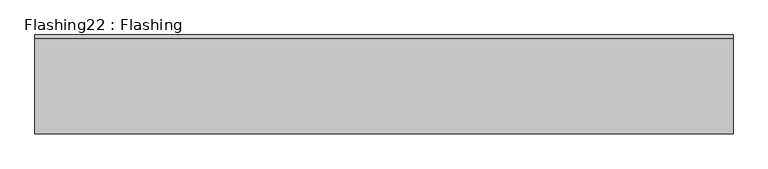
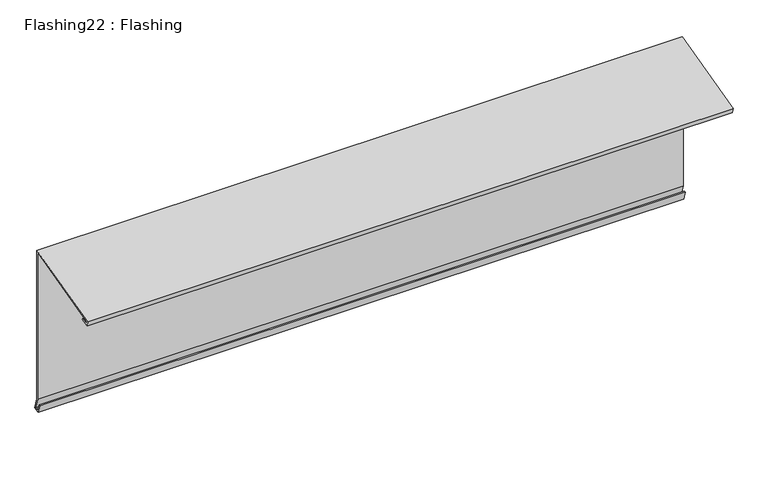
"""IFC4 building model written with IfcOpenShell, lengths in millimetres: proxy geometry, Flashing22 : Flashing."""

from ifc_helpers import new_model, si_unit, frame, origin, place, context, project, spatial, polyline, outline, extrude, source, transform, mapped, element, save


def flashing22_flashing_086f2f6e(model_context):
    return source(origin(), model_context, "Body", "SweptSolid", [
        extrude(outline(polyline([(10550.3613281, 43920.3046875), (10546.9589844, 43935.2734375), (10819.5097656, 44004.90625), (10819.5097656, 43518.7539063), (10830.6904297, 43482.3320313), (10813.1210937, 43476.9648438), (10804.5996094, 43504.4882813), (10808.4206617, 43505.6713107), (10815.7635636, 43481.9545626), (10825.6911014, 43484.9872871), (10815.5097656, 43518.1537731), (10815.5097656, 43999.7558251), (10551.7227627, 43932.3620321), (10553.3654045, 43925.1351625), (10575.0634961, 43930.3201524), (10575.9931641, 43926.4296875), (10550.3613281, 43920.3046875)])), frame((3694.0383192, 0.0, 0.0), z_axis=(1.0, 0.0, 0.0), x_axis=(0.0, 1.0, 0.0)), (0.0, 0.0, 1.0), 2000.25),
    ])


if __name__ == "__main__":
    model = new_model("IFC4")
    model_context = context("Model", 3, world=origin())
    ifc_project = project(units=[si_unit("LENGTHUNIT", "METRE", prefix="MILLI")], contexts=[model_context])
    site = spatial("IfcSite", under=ifc_project)
    building = spatial("IfcBuilding", under=site)
    placement = place(None, origin())
    flashing22_flashing_shape = flashing22_flashing_086f2f6e(model_context)
    element("IfcBuildingElementProxy", 1, Name="Flashing22 : Flashing", ObjectType="Flashing22 : Flashing", at=placement, inside=building, context=model_context, shape_type="MappedRepresentation", body=[
        mapped(flashing22_flashing_shape, transform((0.0, 0.0, 0.0), x_axis=(1.0, 0.0, 0.0), y_axis=(0.0, 1.0, 0.0), z_axis=(0.0, 0.0, 1.0))),
    ])
    save(model, "model.ifc")

# Revit data of these elements
# Type "Flashing22 : Flashing"
#   NameOverride = "Flashing"
# Element 1 (IfcBuildingElementProxy, "Flashing22 : Flashing")
#   Materials on its faces: "BRAKE METAL EAVE TRIM TO MATCH STANDING SEAM COLOR"
# Materials
#   "BRAKE METAL EAVE TRIM TO MATCH STANDING SEAM COLOR": class "Unassigned", colour RGB 128 128 128, transparency 0, Cost = 0
